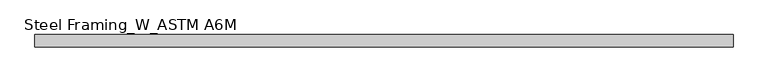
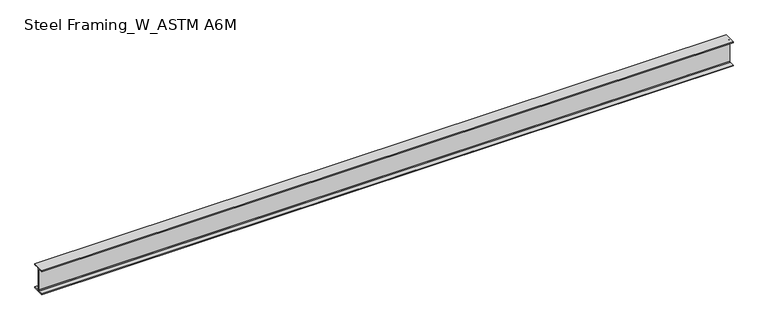
"""IFC4 building model written with IfcOpenShell, lengths in millimetres: beam geometry, Steel Framing_W_ASTM A6M : H_SB_AR_S02_W360x51_B4."""

import ifcopenshell
import ifcopenshell.guid

model = None  # the IFC model being written
_history = None  # IfcOwnerHistory: only IFC2X3 demands one
_inside = {}  # id of a spatial element -> (the spatial element, [elements in it])
_under = {}  # id of a project, library or spatial element -> (it, [spatial elements below it])
_declared = {}  # id of a project -> (the project, [libraries it declares])
_typed = {}  # id of a type object -> (the type object, [elements of that type])
_made_of = {}  # id of a material, layer set ... -> (it, [elements and type objects made of it])


def new_model(schema):
    """Start an empty IFC model of exactly this schema.

    Asked for "IFC4X3", IfcOpenShell would pick the latest addendum, in which some entities
    have other attributes; the version numbers below select the first issue.
    IFC2X3 requires an IfcOwnerHistory on every rooted entity: one is made here for all.
    """
    global model, _history
    if schema == "IFC4X3":
        model = ifcopenshell.file(schema_version=(4, 3, 0, 0))
    else:
        model = ifcopenshell.file(schema=schema)
    _inside.clear()
    _under.clear()
    _declared.clear()
    _typed.clear()
    _made_of.clear()
    _history = None
    if model.schema == "IFC2X3":
        org = make("IfcOrganization", Name="unknown")
        user = make(
            "IfcPersonAndOrganization",
            ThePerson=make("IfcPerson", FamilyName="unknown"),
            TheOrganization=org,
        )
        app = make(
            "IfcApplication",
            ApplicationDeveloper=org,
            Version="unknown",
            ApplicationFullName="unknown",
            ApplicationIdentifier="unknown",
        )
        _history = make(
            "IfcOwnerHistory",
            OwningUser=user,
            OwningApplication=app,
            ChangeAction="ADDED",
            CreationDate=0,
        )
    return model


def make(cls, **values):
    """One entity of the class cls with the attributes given. An attribute that is None is left unset."""
    return model.create_entity(
        cls, **{name: value for name, value in values.items() if value is not None}
    )


def rooted(cls, **values):
    """An entity with a GlobalId (a new one), such as an element, a storey or a relation."""
    return make(cls, GlobalId=ifcopenshell.guid.new(), OwnerHistory=_history, **values)


def si_unit(unit_type, name, prefix=None):
    """IfcSIUnit, for example si_unit("LENGTHUNIT", "METRE", prefix="MILLI")."""
    return make("IfcSIUnit", UnitType=unit_type, Prefix=prefix, Name=name)


def assignment(units):
    """IfcUnitAssignment: the units of a project."""
    return None if units is None else make("IfcUnitAssignment", Units=units)


def point(xyz):
    """IfcCartesianPoint."""
    return None if xyz is None else make("IfcCartesianPoint", Coordinates=xyz)


def direction(xyz):
    """IfcDirection."""
    return None if xyz is None else make("IfcDirection", DirectionRatios=xyz)


def frame(location, z_axis=None, x_axis=None):
    """IfcAxis2Placement3D, a coordinate frame: its origin and axes. An axis left out is left unset."""
    return make(
        "IfcAxis2Placement3D",
        Location=point(location),
        Axis=direction(z_axis),
        RefDirection=direction(x_axis),
    )


def frame_2d(location, x_axis=None):
    """IfcAxis2Placement2D, a coordinate frame in the plane: its origin and x axis."""
    return make(
        "IfcAxis2Placement2D", Location=point(location), RefDirection=direction(x_axis)
    )


def origin():
    """The frame at (0, 0, 0) with its axes left unset."""
    return frame((0.0, 0.0, 0.0))


def place(relative_to, where):
    """IfcLocalPlacement: puts the frame where relative to a parent placement (None: the world)."""
    return make(
        "IfcLocalPlacement", PlacementRelTo=relative_to, RelativePlacement=where
    )


def context(
    kind, dimensions, precision=None, world=None, true_north=None, identifier=None
):
    """IfcGeometricRepresentationContext, for example the 3D "Model" context."""
    return make(
        "IfcGeometricRepresentationContext",
        ContextIdentifier=identifier,
        ContextType=kind,
        CoordinateSpaceDimension=dimensions,
        Precision=precision,
        WorldCoordinateSystem=world,
        TrueNorth=true_north,
    )


def project(units=None, contexts=None):
    """IfcProject with its units and contexts."""
    return rooted(
        "IfcProject",
        Name="project",
        RepresentationContexts=contexts,
        UnitsInContext=assignment(units),
    )


def spatial(cls, under=None, at=None, **own):
    """A site, building, storey or space (cls), placed at a placement, below another one or the project."""
    s = rooted(cls, ObjectPlacement=at, **own)
    if under is not None:
        _under.setdefault(under.id(), (under, []))[1].append(s)
    return s


def polyline(points):
    """IfcPolyline through the points."""
    return make("IfcPolyline", Points=[point(p) for p in points])


def circle_curve(where, radius):
    """IfcCircle in the frame where."""
    return make("IfcCircle", Position=where, Radius=radius)


def trimmed(basis, trim1, trim2, sense, master):
    """IfcTrimmedCurve: the piece of a basis curve between two trims."""
    return make(
        "IfcTrimmedCurve",
        BasisCurve=basis,
        Trim1=trim1,
        Trim2=trim2,
        SenseAgreement=sense,
        MasterRepresentation=master,
    )


def segment(curve, same_sense, transition):
    """IfcCompositeCurveSegment."""
    return make(
        "IfcCompositeCurveSegment",
        Transition=transition,
        SameSense=same_sense,
        ParentCurve=curve,
    )


def composite_curve(segments, self_intersect=None):
    """IfcCompositeCurve: segments joined end to end."""
    return make("IfcCompositeCurve", Segments=segments, SelfIntersect=self_intersect)


def outline(outer, holes=None, kind="AREA"):
    """IfcArbitraryClosedProfileDef: a profile drawn as a closed curve; with holes, ...WithVoids."""
    if holes is None:
        return make("IfcArbitraryClosedProfileDef", ProfileType=kind, OuterCurve=outer)
    return make(
        "IfcArbitraryProfileDefWithVoids",
        ProfileType=kind,
        OuterCurve=outer,
        InnerCurves=holes,
    )


def extrude(swept, where, along, depth):
    """IfcExtrudedAreaSolid: the profile swept, set in the frame where, extruded along a direction by depth."""
    return make(
        "IfcExtrudedAreaSolid",
        SweptArea=swept,
        Position=where,
        ExtrudedDirection=direction(along),
        Depth=depth,
    )


def shape(context_of_items, identifier, shape_type, items):
    """IfcShapeRepresentation: the items that make up one representation, for example the "Body"."""
    return make(
        "IfcShapeRepresentation",
        ContextOfItems=context_of_items,
        RepresentationIdentifier=identifier,
        RepresentationType=shape_type,
        Items=items,
    )


def source(mapping_origin, context_of_items, identifier, shape_type, items):
    """IfcRepresentationMap: a shape defined once, which mapped items show again and again."""
    return make(
        "IfcRepresentationMap",
        MappingOrigin=mapping_origin,
        MappedRepresentation=shape(context_of_items, identifier, shape_type, items),
    )


def transform(
    local_origin,
    x_axis=None,
    y_axis=None,
    z_axis=None,
    scale=None,
    scale2=None,
    scale3=None,
    uniform=True,
):
    """IfcCartesianTransformationOperator3D, or its non-uniform kind. x_axis, y_axis, z_axis: its Axis1, 2, 3."""
    if uniform:
        return make(
            "IfcCartesianTransformationOperator3D",
            Axis1=direction(x_axis),
            Axis2=direction(y_axis),
            LocalOrigin=point(local_origin),
            Scale=scale,
            Axis3=direction(z_axis),
        )
    return make(
        "IfcCartesianTransformationOperator3DnonUniform",
        Axis1=direction(x_axis),
        Axis2=direction(y_axis),
        LocalOrigin=point(local_origin),
        Scale=scale,
        Axis3=direction(z_axis),
        Scale2=scale2,
        Scale3=scale3,
    )


def mapped(mapping_source, mapping_target):
    """IfcMappedItem: shows the shape of a source again, moved by a transform."""
    return make(
        "IfcMappedItem", MappingSource=mapping_source, MappingTarget=mapping_target
    )


def made_of(thing, what):
    """Note that an element or type object is made of a material, layer set ...; save() writes the relation."""
    if what is not None:
        _made_of.setdefault(what.id(), (what, []))[1].append(thing)
    return thing


def element(
    cls,
    number,
    at=None,
    inside=None,
    cuts=None,
    type_object=None,
    material=None,
    context=None,
    identifier="Body",
    shape_type=None,
    held_by="IfcProductDefinitionShape",
    body=None,
    shapes=None,
    **own,
):
    """One element of the class cls, such as IfcWall. Its Tag is "e" and its number.

    at: its placement. inside: the storey or other place that contains it. cuts: it is an
    opening in that element (IfcRelVoidsElement). A single representation is given by context,
    identifier, shape_type and body (its items); several are given by shapes. held_by: the class
    of the entity that holds the representations. save() writes the other relations.
    """
    e = rooted(cls, Tag="e%d" % number, ObjectPlacement=at, **own)
    if body is not None:
        shapes = [shape(context, identifier, shape_type, body)]
    if shapes is not None:
        e.Representation = make(held_by, Representations=shapes)
    if inside is not None:
        _inside.setdefault(inside.id(), (inside, []))[1].append(e)
    if cuts is not None:
        rooted(
            "IfcRelVoidsElement", RelatingBuildingElement=cuts, RelatedOpeningElement=e
        )
    if type_object is not None:
        _typed.setdefault(type_object.id(), (type_object, []))[1].append(e)
    return made_of(e, material)


def aggregate(whole, parts):
    """IfcRelAggregates: a whole, such as a stair, and the parts it consists of."""
    return rooted("IfcRelAggregates", RelatingObject=whole, RelatedObjects=parts)


def save(model, path):
    """Write the relations noted so far, then the file.

    IfcRelAggregates (storeys below a building ...), IfcRelContainedInSpatialStructure (elements
    in a storey), IfcRelDefinesByType, IfcRelAssociatesMaterial and IfcRelDeclares: one each for
    every whole, place, type object, material and project.
    """
    for whole, parts in _under.values():
        aggregate(whole, parts)
    for where, things in _inside.values():
        rooted(
            "IfcRelContainedInSpatialStructure",
            RelatedElements=things,
            RelatingStructure=where,
        )
    for kind, things in _typed.values():
        rooted("IfcRelDefinesByType", RelatedObjects=things, RelatingType=kind)
    for what, things in _made_of.values():
        rooted("IfcRelAssociatesMaterial", RelatedObjects=things, RelatingMaterial=what)
    for by, libraries in _declared.values():
        rooted("IfcRelDeclares", RelatingContext=by, RelatedDefinitions=libraries)
    model.write(path)


def steel_framing_w_astm_a6m_bf6e2db3(model_context):
    return source(origin(), model_context, "Body", "SweptSolid", [
        extrude(outline(composite_curve([segment(polyline([(85.5, -166.4), (85.5, -178.0), (-85.5, -178.0), (-85.5, -166.4), (-13.72, -166.4)]), True, "CONTINUOUS"), segment(trimmed(circle_curve(frame_2d((-13.72, -156.3)), 10.1), [point((-13.72, -166.4))], [point((-3.62, -156.3))], True, "CARTESIAN"), True, "CONTINUOUS"), segment(polyline([(-3.62, -156.3), (-3.62, 156.3)]), True, "CONTINUOUS"), segment(trimmed(circle_curve(frame_2d((-13.72, 156.3)), 10.1), [point((-3.62, 156.3))], [point((-13.72, 166.4))], True, "CARTESIAN"), True, "CONTINUOUS"), segment(polyline([(-13.72, 166.4), (-85.5, 166.4), (-85.5, 178.0), (85.5, 178.0), (85.5, 166.4), (13.72, 166.4)]), True, "CONTINUOUS"), segment(trimmed(circle_curve(frame_2d((13.72, 156.3)), 10.1), [point((13.72, 166.4))], [point((3.62, 156.3))], True, "CARTESIAN"), True, "CONTINUOUS"), segment(polyline([(3.62, 156.3), (3.62, -156.3)]), True, "CONTINUOUS"), segment(trimmed(circle_curve(frame_2d((13.72, -156.3)), 10.1), [point((3.62, -156.3))], [point((13.72, -166.4))], True, "CARTESIAN"), True, "CONTINUOUS"), segment(polyline([(13.72, -166.4), (85.5, -166.4)]), True, "CONTINUOUS")], self_intersect=False)), frame((-4814.1, 0.0, 0.0), z_axis=(1.0, 0.0, 0.0), x_axis=(0.0, 1.0, 0.0)), (0.0, 0.0, 1.0), 9715.9),
    ])


if __name__ == "__main__":
    model = new_model("IFC4")
    model_context = context("Model", 3, world=origin())
    ifc_project = project(units=[si_unit("LENGTHUNIT", "METRE", prefix="MILLI")], contexts=[model_context])
    site = spatial("IfcSite", under=ifc_project)
    building = spatial("IfcBuilding", under=site)
    placement = place(None, origin())
    steel_framing_w_astm_a6m_shape = steel_framing_w_astm_a6m_bf6e2db3(model_context)
    element("IfcBeam", 1, ObjectType="Steel Framing_W_ASTM A6M : H_SB_AR_S02_W360x51_B4", at=placement, inside=building, context=model_context, shape_type="MappedRepresentation", body=[
        mapped(steel_framing_w_astm_a6m_shape, transform((0.0, 0.0, 0.0), x_axis=(1.0, 0.0, 0.0), y_axis=(0.0, 1.0, 0.0), z_axis=(0.0, 0.0, 1.0))),
    ])
    save(model, "model.ifc")

# Revit data of these elements
# Type "Steel Framing_W_ASTM A6M : H_SB_AR_S02_W360x51_B4"
#   Type Mark = "B4"
#   Section Name Key = "W14x34"
#   Width = 17.1 cm
#   Web Thickness = 0.724 cm
#   Web Fillet = 1.01 cm
#   Warping Constant = 287000.0 cm⁶
#   Torsional Moment of Inertia = 23.70 cm⁴
#   Section Area = 64.5 cm²
#   Plastic Modulus weak axis = 174.0 cm³
#   Plastic Modulus strong axis = 895.0 cm³
#   Perimeter = 1.36 m²/m
#   Nominal Weight = 51.00 kgf/m
#   Moment of Inertia weak axis = 970.00 cm⁴
#   Moment of Inertia strong axis = 14200.00 cm⁴
#   Height = 35.6 cm
#   Flange Thickness = 1.16 cm
#   Elastic Modulus weak axis = 113.0 cm³
#   Elastic Modulus strong axis = 796.0 cm³
#   Centroid Vertical = 17.8 cm
#   Centroid Horizontal = 8.55 cm
#   Length [instance default] = 1500 mm
#   Structural Material [instance default] = Steel, 45-345
#   Bolt Spacing = 0
#   Assembly Code = ""
# Element 1 (IfcBeam, "Steel Framing_W_ASTM A6M : H_SB_AR_S02_W360x51_B4")
#   Materials on its faces: "Steel, 45-345"
# Materials
#   "Steel, 45-345": class "Metal", colour RGB 189 187 185, transparency 0, Description = "Steel 345 MPa", Cost = 0
